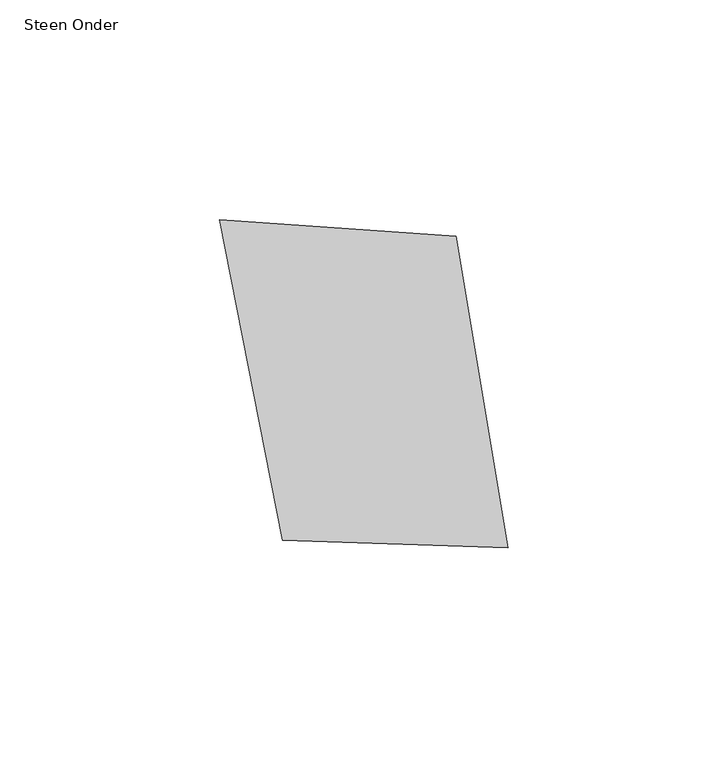
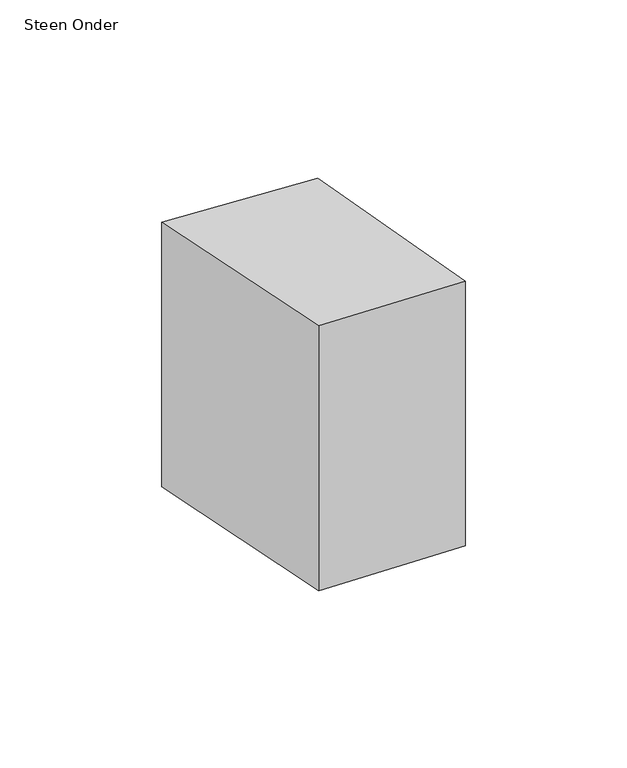
"""IFC4 building model written with IfcOpenShell, lengths in millimetres: proxy geometry, 00_GMA_steen_versie_4 : Steen Onder."""

import ifcopenshell
import ifcopenshell.guid

model = None  # the IFC model being written
_history = None  # IfcOwnerHistory: only IFC2X3 demands one
_inside = {}  # id of a spatial element -> (the spatial element, [elements in it])
_under = {}  # id of a project, library or spatial element -> (it, [spatial elements below it])
_declared = {}  # id of a project -> (the project, [libraries it declares])
_typed = {}  # id of a type object -> (the type object, [elements of that type])
_made_of = {}  # id of a material, layer set ... -> (it, [elements and type objects made of it])


def new_model(schema):
    """Start an empty IFC model of exactly this schema.

    Asked for "IFC4X3", IfcOpenShell would pick the latest addendum, in which some entities
    have other attributes; the version numbers below select the first issue.
    IFC2X3 requires an IfcOwnerHistory on every rooted entity: one is made here for all.
    """
    global model, _history
    if schema == "IFC4X3":
        model = ifcopenshell.file(schema_version=(4, 3, 0, 0))
    else:
        model = ifcopenshell.file(schema=schema)
    _inside.clear()
    _under.clear()
    _declared.clear()
    _typed.clear()
    _made_of.clear()
    _history = None
    if model.schema == "IFC2X3":
        org = make("IfcOrganization", Name="unknown")
        user = make(
            "IfcPersonAndOrganization",
            ThePerson=make("IfcPerson", FamilyName="unknown"),
            TheOrganization=org,
        )
        app = make(
            "IfcApplication",
            ApplicationDeveloper=org,
            Version="unknown",
            ApplicationFullName="unknown",
            ApplicationIdentifier="unknown",
        )
        _history = make(
            "IfcOwnerHistory",
            OwningUser=user,
            OwningApplication=app,
            ChangeAction="ADDED",
            CreationDate=0,
        )
    return model


def make(cls, **values):
    """One entity of the class cls with the attributes given. An attribute that is None is left unset."""
    return model.create_entity(
        cls, **{name: value for name, value in values.items() if value is not None}
    )


def rooted(cls, **values):
    """An entity with a GlobalId (a new one), such as an element, a storey or a relation."""
    return make(cls, GlobalId=ifcopenshell.guid.new(), OwnerHistory=_history, **values)


def si_unit(unit_type, name, prefix=None):
    """IfcSIUnit, for example si_unit("LENGTHUNIT", "METRE", prefix="MILLI")."""
    return make("IfcSIUnit", UnitType=unit_type, Prefix=prefix, Name=name)


def assignment(units):
    """IfcUnitAssignment: the units of a project."""
    return None if units is None else make("IfcUnitAssignment", Units=units)


def point(xyz):
    """IfcCartesianPoint."""
    return None if xyz is None else make("IfcCartesianPoint", Coordinates=xyz)


def direction(xyz):
    """IfcDirection."""
    return None if xyz is None else make("IfcDirection", DirectionRatios=xyz)


def frame(location, z_axis=None, x_axis=None):
    """IfcAxis2Placement3D, a coordinate frame: its origin and axes. An axis left out is left unset."""
    return make(
        "IfcAxis2Placement3D",
        Location=point(location),
        Axis=direction(z_axis),
        RefDirection=direction(x_axis),
    )


def origin():
    """The frame at (0, 0, 0) with its axes left unset."""
    return frame((0.0, 0.0, 0.0))


def origin_with_axes():
    """The frame at (0, 0, 0) with the z axis (0, 0, 1) and the x axis (1, 0, 0) written out."""
    return frame((0.0, 0.0, 0.0), z_axis=(0.0, 0.0, 1.0), x_axis=(1.0, 0.0, 0.0))


def place(relative_to, where):
    """IfcLocalPlacement: puts the frame where relative to a parent placement (None: the world)."""
    return make(
        "IfcLocalPlacement", PlacementRelTo=relative_to, RelativePlacement=where
    )


def context(
    kind, dimensions, precision=None, world=None, true_north=None, identifier=None
):
    """IfcGeometricRepresentationContext, for example the 3D "Model" context."""
    return make(
        "IfcGeometricRepresentationContext",
        ContextIdentifier=identifier,
        ContextType=kind,
        CoordinateSpaceDimension=dimensions,
        Precision=precision,
        WorldCoordinateSystem=world,
        TrueNorth=true_north,
    )


def project(units=None, contexts=None):
    """IfcProject with its units and contexts."""
    return rooted(
        "IfcProject",
        Name="project",
        RepresentationContexts=contexts,
        UnitsInContext=assignment(units),
    )


def spatial(cls, under=None, at=None, **own):
    """A site, building, storey or space (cls), placed at a placement, below another one or the project."""
    s = rooted(cls, ObjectPlacement=at, **own)
    if under is not None:
        _under.setdefault(under.id(), (under, []))[1].append(s)
    return s


def polyline(points):
    """IfcPolyline through the points."""
    return make("IfcPolyline", Points=[point(p) for p in points])


def outline(outer, holes=None, kind="AREA"):
    """IfcArbitraryClosedProfileDef: a profile drawn as a closed curve; with holes, ...WithVoids."""
    if holes is None:
        return make("IfcArbitraryClosedProfileDef", ProfileType=kind, OuterCurve=outer)
    return make(
        "IfcArbitraryProfileDefWithVoids",
        ProfileType=kind,
        OuterCurve=outer,
        InnerCurves=holes,
    )


def extrude(swept, where, along, depth):
    """IfcExtrudedAreaSolid: the profile swept, set in the frame where, extruded along a direction by depth."""
    return make(
        "IfcExtrudedAreaSolid",
        SweptArea=swept,
        Position=where,
        ExtrudedDirection=direction(along),
        Depth=depth,
    )


def shape(context_of_items, identifier, shape_type, items):
    """IfcShapeRepresentation: the items that make up one representation, for example the "Body"."""
    return make(
        "IfcShapeRepresentation",
        ContextOfItems=context_of_items,
        RepresentationIdentifier=identifier,
        RepresentationType=shape_type,
        Items=items,
    )


def source(mapping_origin, context_of_items, identifier, shape_type, items):
    """IfcRepresentationMap: a shape defined once, which mapped items show again and again."""
    return make(
        "IfcRepresentationMap",
        MappingOrigin=mapping_origin,
        MappedRepresentation=shape(context_of_items, identifier, shape_type, items),
    )


def transform(
    local_origin,
    x_axis=None,
    y_axis=None,
    z_axis=None,
    scale=None,
    scale2=None,
    scale3=None,
    uniform=True,
):
    """IfcCartesianTransformationOperator3D, or its non-uniform kind. x_axis, y_axis, z_axis: its Axis1, 2, 3."""
    if uniform:
        return make(
            "IfcCartesianTransformationOperator3D",
            Axis1=direction(x_axis),
            Axis2=direction(y_axis),
            LocalOrigin=point(local_origin),
            Scale=scale,
            Axis3=direction(z_axis),
        )
    return make(
        "IfcCartesianTransformationOperator3DnonUniform",
        Axis1=direction(x_axis),
        Axis2=direction(y_axis),
        LocalOrigin=point(local_origin),
        Scale=scale,
        Axis3=direction(z_axis),
        Scale2=scale2,
        Scale3=scale3,
    )


def mapped(mapping_source, mapping_target):
    """IfcMappedItem: shows the shape of a source again, moved by a transform."""
    return make(
        "IfcMappedItem", MappingSource=mapping_source, MappingTarget=mapping_target
    )


def made_of(thing, what):
    """Note that an element or type object is made of a material, layer set ...; save() writes the relation."""
    if what is not None:
        _made_of.setdefault(what.id(), (what, []))[1].append(thing)
    return thing


def element(
    cls,
    number,
    at=None,
    inside=None,
    cuts=None,
    type_object=None,
    material=None,
    context=None,
    identifier="Body",
    shape_type=None,
    held_by="IfcProductDefinitionShape",
    body=None,
    shapes=None,
    **own,
):
    """One element of the class cls, such as IfcWall. Its Tag is "e" and its number.

    at: its placement. inside: the storey or other place that contains it. cuts: it is an
    opening in that element (IfcRelVoidsElement). A single representation is given by context,
    identifier, shape_type and body (its items); several are given by shapes. held_by: the class
    of the entity that holds the representations. save() writes the other relations.
    """
    e = rooted(cls, Tag="e%d" % number, ObjectPlacement=at, **own)
    if body is not None:
        shapes = [shape(context, identifier, shape_type, body)]
    if shapes is not None:
        e.Representation = make(held_by, Representations=shapes)
    if inside is not None:
        _inside.setdefault(inside.id(), (inside, []))[1].append(e)
    if cuts is not None:
        rooted(
            "IfcRelVoidsElement", RelatingBuildingElement=cuts, RelatedOpeningElement=e
        )
    if type_object is not None:
        _typed.setdefault(type_object.id(), (type_object, []))[1].append(e)
    return made_of(e, material)


def aggregate(whole, parts):
    """IfcRelAggregates: a whole, such as a stair, and the parts it consists of."""
    return rooted("IfcRelAggregates", RelatingObject=whole, RelatedObjects=parts)


def save(model, path):
    """Write the relations noted so far, then the file.

    IfcRelAggregates (storeys below a building ...), IfcRelContainedInSpatialStructure (elements
    in a storey), IfcRelDefinesByType, IfcRelAssociatesMaterial and IfcRelDeclares: one each for
    every whole, place, type object, material and project.
    """
    for whole, parts in _under.values():
        aggregate(whole, parts)
    for where, things in _inside.values():
        rooted(
            "IfcRelContainedInSpatialStructure",
            RelatedElements=things,
            RelatingStructure=where,
        )
    for kind, things in _typed.values():
        rooted("IfcRelDefinesByType", RelatedObjects=things, RelatingType=kind)
    for what, things in _made_of.values():
        rooted("IfcRelAssociatesMaterial", RelatedObjects=things, RelatingMaterial=what)
    for by, libraries in _declared.values():
        rooted("IfcRelDeclares", RelatingContext=by, RelatedDefinitions=libraries)
    model.write(path)


def steen_onder_a90a9219(model_context):
    return source(origin(), model_context, "Body", "SweptSolid", [
        extrude(outline(polyline([(95.102577, 101.8678488), (106.8413547, 31.0004019), (55.576017, 32.7038157), (41.3613936, 105.5435647), (95.102577, 101.8678488)])), origin_with_axes(), (0.0, 0.0, 1.0), 100.0),
    ])


if __name__ == "__main__":
    model = new_model("IFC4")
    model_context = context("Model", 3, world=origin())
    ifc_project = project(units=[si_unit("LENGTHUNIT", "METRE", prefix="MILLI")], contexts=[model_context])
    site = spatial("IfcSite", under=ifc_project)
    building = spatial("IfcBuilding", under=site)
    placement = place(None, origin())
    steen_onder_shape = steen_onder_a90a9219(model_context)
    element("IfcBuildingElementProxy", 1, Name="00_GMA_steen_versie_4 : Steen Onder", ObjectType="00_GMA_steen_versie_4 : Steen Onder", at=placement, inside=building, context=model_context, shape_type="MappedRepresentation", body=[
        mapped(steen_onder_shape, transform((0.0, 0.0, 0.0), x_axis=(1.0, 0.0, 0.0), y_axis=(0.0, 1.0, 0.0), z_axis=(0.0, 0.0, 1.0))),
    ])
    save(model, "model.ifc")

# Revit data of these elements
# Type "00_GMA_steen_versie_4 : Steen Onder"
#   StootVoegHalfBoven [instance default] = 5 mm
#   StootVoegHalf [instance default] = 5 mm
#   StootVoegBreedteOnder = 10 mm
#   StootVoegBreedteBoven = 10 mm
#   Steendikte = 100 mm
#   LintVoegOnderHalf = 0 mm
#   LintVoegOnder = 0 mm
#   LintVoegBovenHalf = 5 mm
#   LintVoegBoven = 10 mm
#   materiaal = none
#   MateriaalVoeg = none
#   Default Elevation = 0
